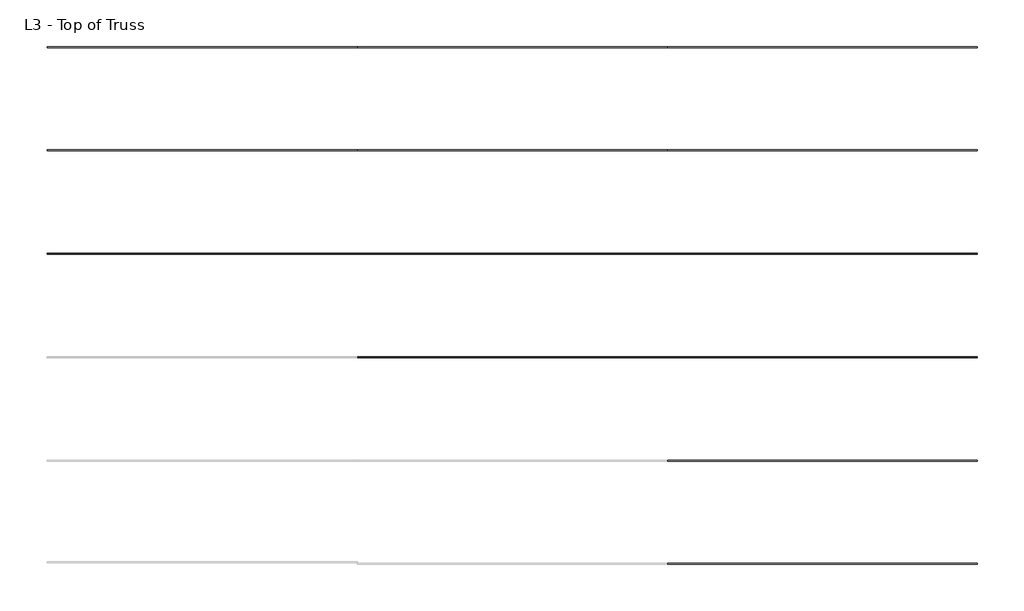
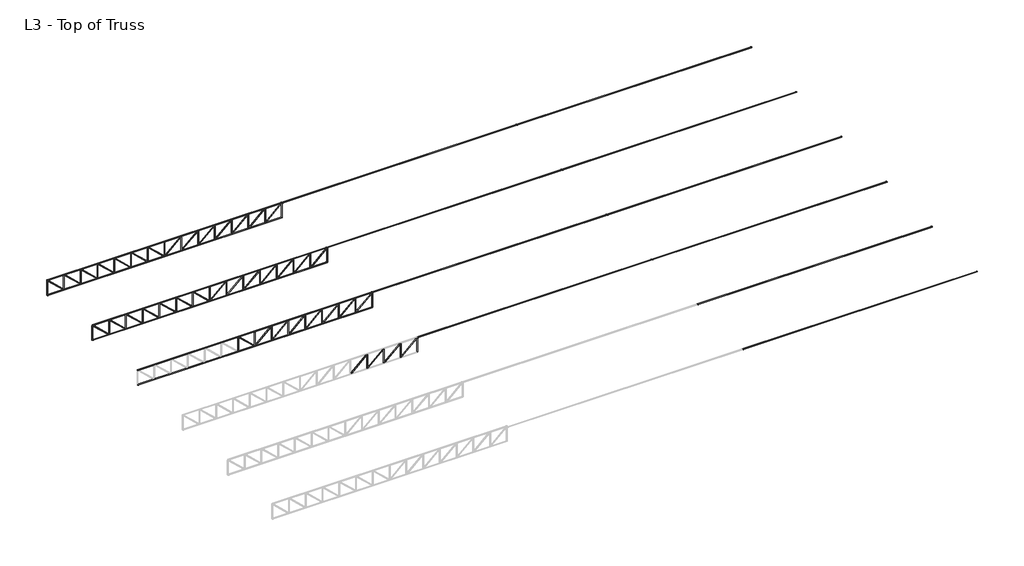
# One storey, part 2 of 2: 100 beams.
"""IFC4 building model written with IfcOpenShell, lengths in millimetres."""

import ifcopenshell
import ifcopenshell.guid

model = None  # the IFC model being written
_history = None  # IfcOwnerHistory: only IFC2X3 demands one
_inside = {}  # id of a spatial element -> (the spatial element, [elements in it])
_under = {}  # id of a project, library or spatial element -> (it, [spatial elements below it])
_declared = {}  # id of a project -> (the project, [libraries it declares])
_typed = {}  # id of a type object -> (the type object, [elements of that type])
_made_of = {}  # id of a material, layer set ... -> (it, [elements and type objects made of it])


def new_model(schema):
    """Start an empty IFC model of exactly this schema.

    Asked for "IFC4X3", IfcOpenShell would pick the latest addendum, in which some entities
    have other attributes; the version numbers below select the first issue.
    IFC2X3 requires an IfcOwnerHistory on every rooted entity: one is made here for all.
    """
    global model, _history
    if schema == "IFC4X3":
        model = ifcopenshell.file(schema_version=(4, 3, 0, 0))
    else:
        model = ifcopenshell.file(schema=schema)
    _inside.clear()
    _under.clear()
    _declared.clear()
    _typed.clear()
    _made_of.clear()
    _history = None
    if model.schema == "IFC2X3":
        org = make("IfcOrganization", Name="unknown")
        user = make(
            "IfcPersonAndOrganization",
            ThePerson=make("IfcPerson", FamilyName="unknown"),
            TheOrganization=org,
        )
        app = make(
            "IfcApplication",
            ApplicationDeveloper=org,
            Version="unknown",
            ApplicationFullName="unknown",
            ApplicationIdentifier="unknown",
        )
        _history = make(
            "IfcOwnerHistory",
            OwningUser=user,
            OwningApplication=app,
            ChangeAction="ADDED",
            CreationDate=0,
        )
    return model


def make(cls, **values):
    """One entity of the class cls with the attributes given. An attribute that is None is left unset."""
    return model.create_entity(
        cls, **{name: value for name, value in values.items() if value is not None}
    )


def rooted(cls, **values):
    """An entity with a GlobalId (a new one), such as an element, a storey or a relation."""
    return make(cls, GlobalId=ifcopenshell.guid.new(), OwnerHistory=_history, **values)


def si_unit(unit_type, name, prefix=None):
    """IfcSIUnit, for example si_unit("LENGTHUNIT", "METRE", prefix="MILLI")."""
    return make("IfcSIUnit", UnitType=unit_type, Prefix=prefix, Name=name)


def assignment(units):
    """IfcUnitAssignment: the units of a project."""
    return None if units is None else make("IfcUnitAssignment", Units=units)


def point(xyz):
    """IfcCartesianPoint."""
    return None if xyz is None else make("IfcCartesianPoint", Coordinates=xyz)


def direction(xyz):
    """IfcDirection."""
    return None if xyz is None else make("IfcDirection", DirectionRatios=xyz)


def frame(location, z_axis=None, x_axis=None):
    """IfcAxis2Placement3D, a coordinate frame: its origin and axes. An axis left out is left unset."""
    return make(
        "IfcAxis2Placement3D",
        Location=point(location),
        Axis=direction(z_axis),
        RefDirection=direction(x_axis),
    )


def frame_2d(location, x_axis=None):
    """IfcAxis2Placement2D, a coordinate frame in the plane: its origin and x axis."""
    return make(
        "IfcAxis2Placement2D", Location=point(location), RefDirection=direction(x_axis)
    )


def origin():
    """The frame at (0, 0, 0) with its axes left unset."""
    return frame((0.0, 0.0, 0.0))


def origin_2d():
    """The frame at (0, 0) in the plane with its x axis left unset."""
    return frame_2d((0.0, 0.0))


def place(relative_to, where):
    """IfcLocalPlacement: puts the frame where relative to a parent placement (None: the world)."""
    return make(
        "IfcLocalPlacement", PlacementRelTo=relative_to, RelativePlacement=where
    )


def context(
    kind, dimensions, precision=None, world=None, true_north=None, identifier=None
):
    """IfcGeometricRepresentationContext, for example the 3D "Model" context."""
    return make(
        "IfcGeometricRepresentationContext",
        ContextIdentifier=identifier,
        ContextType=kind,
        CoordinateSpaceDimension=dimensions,
        Precision=precision,
        WorldCoordinateSystem=world,
        TrueNorth=true_north,
    )


def project(units=None, contexts=None):
    """IfcProject with its units and contexts."""
    return rooted(
        "IfcProject",
        Name="project",
        RepresentationContexts=contexts,
        UnitsInContext=assignment(units),
    )


def spatial(cls, under=None, at=None, **own):
    """A site, building, storey or space (cls), placed at a placement, below another one or the project."""
    s = rooted(cls, ObjectPlacement=at, **own)
    if under is not None:
        _under.setdefault(under.id(), (under, []))[1].append(s)
    return s


def circle_curve(where, radius):
    """IfcCircle in the frame where."""
    return make("IfcCircle", Position=where, Radius=radius)


def trimmed(basis, trim1, trim2, sense, master):
    """IfcTrimmedCurve: the piece of a basis curve between two trims."""
    return make(
        "IfcTrimmedCurve",
        BasisCurve=basis,
        Trim1=trim1,
        Trim2=trim2,
        SenseAgreement=sense,
        MasterRepresentation=master,
    )


def segment(curve, same_sense, transition):
    """IfcCompositeCurveSegment."""
    return make(
        "IfcCompositeCurveSegment",
        Transition=transition,
        SameSense=same_sense,
        ParentCurve=curve,
    )


def composite_curve(segments, self_intersect=None):
    """IfcCompositeCurve: segments joined end to end."""
    return make("IfcCompositeCurve", Segments=segments, SelfIntersect=self_intersect)


def outline(outer, holes=None, kind="AREA"):
    """IfcArbitraryClosedProfileDef: a profile drawn as a closed curve; with holes, ...WithVoids."""
    if holes is None:
        return make("IfcArbitraryClosedProfileDef", ProfileType=kind, OuterCurve=outer)
    return make(
        "IfcArbitraryProfileDefWithVoids",
        ProfileType=kind,
        OuterCurve=outer,
        InnerCurves=holes,
    )


def extrude(swept, where, along, depth):
    """IfcExtrudedAreaSolid: the profile swept, set in the frame where, extruded along a direction by depth."""
    return make(
        "IfcExtrudedAreaSolid",
        SweptArea=swept,
        Position=where,
        ExtrudedDirection=direction(along),
        Depth=depth,
    )


def shape(context_of_items, identifier, shape_type, items):
    """IfcShapeRepresentation: the items that make up one representation, for example the "Body"."""
    return make(
        "IfcShapeRepresentation",
        ContextOfItems=context_of_items,
        RepresentationIdentifier=identifier,
        RepresentationType=shape_type,
        Items=items,
    )


def source(mapping_origin, context_of_items, identifier, shape_type, items):
    """IfcRepresentationMap: a shape defined once, which mapped items show again and again."""
    return make(
        "IfcRepresentationMap",
        MappingOrigin=mapping_origin,
        MappedRepresentation=shape(context_of_items, identifier, shape_type, items),
    )


def transform(
    local_origin,
    x_axis=None,
    y_axis=None,
    z_axis=None,
    scale=None,
    scale2=None,
    scale3=None,
    uniform=True,
):
    """IfcCartesianTransformationOperator3D, or its non-uniform kind. x_axis, y_axis, z_axis: its Axis1, 2, 3."""
    if uniform:
        return make(
            "IfcCartesianTransformationOperator3D",
            Axis1=direction(x_axis),
            Axis2=direction(y_axis),
            LocalOrigin=point(local_origin),
            Scale=scale,
            Axis3=direction(z_axis),
        )
    return make(
        "IfcCartesianTransformationOperator3DnonUniform",
        Axis1=direction(x_axis),
        Axis2=direction(y_axis),
        LocalOrigin=point(local_origin),
        Scale=scale,
        Axis3=direction(z_axis),
        Scale2=scale2,
        Scale3=scale3,
    )


def mapped(mapping_source, mapping_target):
    """IfcMappedItem: shows the shape of a source again, moved by a transform."""
    return make(
        "IfcMappedItem", MappingSource=mapping_source, MappingTarget=mapping_target
    )


def made_of(thing, what):
    """Note that an element or type object is made of a material, layer set ...; save() writes the relation."""
    if what is not None:
        _made_of.setdefault(what.id(), (what, []))[1].append(thing)
    return thing


def element(
    cls,
    number,
    at=None,
    inside=None,
    cuts=None,
    type_object=None,
    material=None,
    context=None,
    identifier="Body",
    shape_type=None,
    held_by="IfcProductDefinitionShape",
    body=None,
    shapes=None,
    **own,
):
    """One element of the class cls, such as IfcWall. Its Tag is "e" and its number.

    at: its placement. inside: the storey or other place that contains it. cuts: it is an
    opening in that element (IfcRelVoidsElement). A single representation is given by context,
    identifier, shape_type and body (its items); several are given by shapes. held_by: the class
    of the entity that holds the representations. save() writes the other relations.
    """
    e = rooted(cls, Tag="e%d" % number, ObjectPlacement=at, **own)
    if body is not None:
        shapes = [shape(context, identifier, shape_type, body)]
    if shapes is not None:
        e.Representation = make(held_by, Representations=shapes)
    if inside is not None:
        _inside.setdefault(inside.id(), (inside, []))[1].append(e)
    if cuts is not None:
        rooted(
            "IfcRelVoidsElement", RelatingBuildingElement=cuts, RelatedOpeningElement=e
        )
    if type_object is not None:
        _typed.setdefault(type_object.id(), (type_object, []))[1].append(e)
    return made_of(e, material)


def aggregate(whole, parts):
    """IfcRelAggregates: a whole, such as a stair, and the parts it consists of."""
    return rooted("IfcRelAggregates", RelatingObject=whole, RelatedObjects=parts)


def save(model, path):
    """Write the relations noted so far, then the file.

    IfcRelAggregates (storeys below a building ...), IfcRelContainedInSpatialStructure (elements
    in a storey), IfcRelDefinesByType, IfcRelAssociatesMaterial and IfcRelDeclares: one each for
    every whole, place, type object, material and project.
    """
    for whole, parts in _under.values():
        aggregate(whole, parts)
    for where, things in _inside.values():
        rooted(
            "IfcRelContainedInSpatialStructure",
            RelatedElements=things,
            RelatingStructure=where,
        )
    for kind, things in _typed.values():
        rooted("IfcRelDefinesByType", RelatedObjects=things, RelatingType=kind)
    for what, things in _made_of.values():
        rooted("IfcRelAssociatesMaterial", RelatedObjects=things, RelatingMaterial=what)
    for by, libraries in _declared.values():
        rooted("IfcRelDeclares", RelatingContext=by, RelatedDefinitions=libraries)
    model.write(path)


def circular_hollow_sections_chs60_3x5_c94bd862(model_context):
    return source(origin(), model_context, "Body", "SweptSolid", [
        extrude(outline(composite_curve([segment(trimmed(circle_curve(origin_2d(), 30.15), [point((-30.15, 0.0))], [point((30.15, 0.0))], False, "CARTESIAN"), True, "CONTINUOUS"), segment(trimmed(circle_curve(origin_2d(), 30.15), [point((30.15, 0.0))], [point((-30.15, 0.0))], False, "CARTESIAN"), True, "CONTINUOUS")], self_intersect=False), holes=[composite_curve([segment(trimmed(circle_curve(origin_2d(), 25.15), [point((25.15, 0.0))], [point((-25.15, 0.0))], True, "CARTESIAN"), True, "CONTINUOUS"), segment(trimmed(circle_curve(origin_2d(), 25.15), [point((-25.15, 0.0))], [point((25.15, 0.0))], True, "CARTESIAN"), True, "CONTINUOUS")], self_intersect=False)]), frame((-557.0, 0.0, 0.0), z_axis=(1.0, 0.0, 0.0), x_axis=(0.0, 1.0, 0.0)), (0.0, 0.0, 1.0), 1114.0),
    ])


def circular_hollow_sections_chs60_3x5_b8a643cb(model_context):
    return source(origin(), model_context, "Body", "SweptSolid", [
        extrude(outline(composite_curve([segment(trimmed(circle_curve(origin_2d(), 30.15), [point((-30.15, 0.0))], [point((30.15, 0.0))], False, "CARTESIAN"), True, "CONTINUOUS"), segment(trimmed(circle_curve(origin_2d(), 30.15), [point((30.15, 0.0))], [point((-30.15, 0.0))], False, "CARTESIAN"), True, "CONTINUOUS")], self_intersect=False), holes=[composite_curve([segment(trimmed(circle_curve(origin_2d(), 25.15), [point((25.15, 0.0))], [point((-25.15, 0.0))], True, "CARTESIAN"), True, "CONTINUOUS"), segment(trimmed(circle_curve(origin_2d(), 25.15), [point((-25.15, 0.0))], [point((25.15, 0.0))], True, "CARTESIAN"), True, "CONTINUOUS")], self_intersect=False)]), frame((-790.0, 0.0, 0.0), z_axis=(1.0, 0.0, 0.0), x_axis=(0.0, 1.0, 0.0)), (0.0, 0.0, 1.0), 1580.0),
    ])


def circular_hollow_sections_chs60_3x5_ee2473de(model_context):
    return source(origin(), model_context, "Body", "SweptSolid", [
        extrude(outline(composite_curve([segment(trimmed(circle_curve(origin_2d(), 30.15), [point((-30.15, 0.0))], [point((30.15, 0.0))], False, "CARTESIAN"), True, "CONTINUOUS"), segment(trimmed(circle_curve(origin_2d(), 30.15), [point((30.15, 0.0))], [point((-30.15, 0.0))], False, "CARTESIAN"), True, "CONTINUOUS")], self_intersect=False), holes=[composite_curve([segment(trimmed(circle_curve(origin_2d(), 25.15), [point((25.15, 0.0))], [point((-25.15, 0.0))], True, "CARTESIAN"), True, "CONTINUOUS"), segment(trimmed(circle_curve(origin_2d(), 25.15), [point((-25.15, 0.0))], [point((25.15, 0.0))], True, "CARTESIAN"), True, "CONTINUOUS")], self_intersect=False)]), frame((-9000.0, 0.0, 0.0), z_axis=(1.0, 0.0, 0.0), x_axis=(0.0, 1.0, 0.0)), (0.0, 0.0, 1.0), 18000.0),
    ])


def circular_hollow_sections_chs60_3x5_7809bf4e(model_context):
    return source(origin(), model_context, "Body", "SweptSolid", [
        extrude(outline(composite_curve([segment(trimmed(circle_curve(origin_2d(), 30.15), [point((-30.15, 0.0))], [point((30.15, 0.0))], False, "CARTESIAN"), True, "CONTINUOUS"), segment(trimmed(circle_curve(origin_2d(), 30.15), [point((30.15, 0.0))], [point((-30.15, 0.0))], False, "CARTESIAN"), True, "CONTINUOUS")], self_intersect=False), holes=[composite_curve([segment(trimmed(circle_curve(origin_2d(), 25.15), [point((25.15, 0.0))], [point((-25.15, 0.0))], True, "CARTESIAN"), True, "CONTINUOUS"), segment(trimmed(circle_curve(origin_2d(), 25.15), [point((-25.15, 0.0))], [point((25.15, 0.0))], True, "CARTESIAN"), True, "CONTINUOUS")], self_intersect=False)]), frame((-600.0, 0.0, 0.0), z_axis=(1.0, 0.0, 0.0), x_axis=(0.0, 1.0, 0.0)), (0.0, 0.0, 1.0), 1157.0),
    ])


model = new_model("IFC4")

# Units and contexts
model_context = context("Model", 3, world=origin())
ifc_project = project(units=[si_unit("LENGTHUNIT", "METRE", prefix="MILLI")], contexts=[model_context])

# Site, building, storey
site = spatial("IfcSite", under=ifc_project)
building = spatial("IfcBuilding", under=site)
storey = spatial("IfcBuildingStorey", under=building, Name="L3 - Top of Truss", Elevation=7800.0)

# Beams
placement = place(None, origin())
circular_hollow_sections_chs60_3x5_shape = circular_hollow_sections_chs60_3x5_c94bd862(model_context)
element("IfcBeam", 1, ObjectType="Circular Hollow Sections : CHS60.3x5", at=placement, inside=storey, context=model_context, shape_type="MappedRepresentation", body=[
    mapped(circular_hollow_sections_chs60_3x5_shape, transform((9574.7303686, 941.2380918, 7200.0), x_axis=(0.0, 0.0, 1.0), y_axis=(0.0, -1.0, 0.0), z_axis=(1.0, 0.0, 0.0))),
])
element("IfcBeam", 2, ObjectType="Circular Hollow Sections : CHS60.3x5", at=placement, inside=storey, context=model_context, shape_type="MappedRepresentation", body=[
    mapped(circular_hollow_sections_chs60_3x5_shape, transform((-5853.84106, 941.2380918, 7200.0), x_axis=(0.0, 0.0, 1.0), y_axis=(0.0, -1.0, 0.0), z_axis=(1.0, 0.0, 0.0))),
])
element("IfcBeam", 3, ObjectType="Circular Hollow Sections : CHS60.3x5", at=placement, inside=storey, context=model_context, shape_type="MappedRepresentation", body=[
    mapped(circular_hollow_sections_chs60_3x5_shape, transform((8289.0160829, 941.2380918, 7200.0), x_axis=(0.0, 0.0, 1.0), y_axis=(0.0, -1.0, 0.0), z_axis=(1.0, 0.0, 0.0))),
])
element("IfcBeam", 4, ObjectType="Circular Hollow Sections : CHS60.3x5", at=placement, inside=storey, context=model_context, shape_type="MappedRepresentation", body=[
    mapped(circular_hollow_sections_chs60_3x5_shape, transform((-4568.1267743, 941.2380918, 7200.0), x_axis=(0.0, 0.0, 1.0), y_axis=(0.0, -1.0, 0.0), z_axis=(1.0, 0.0, 0.0))),
])
element("IfcBeam", 5, ObjectType="Circular Hollow Sections : CHS60.3x5", at=placement, inside=storey, context=model_context, shape_type="MappedRepresentation", body=[
    mapped(circular_hollow_sections_chs60_3x5_shape, transform((7003.3017972, 941.2380918, 7200.0), x_axis=(0.0, 0.0, 1.0), y_axis=(0.0, -1.0, 0.0), z_axis=(1.0, 0.0, 0.0))),
])
element("IfcBeam", 6, ObjectType="Circular Hollow Sections : CHS60.3x5", at=placement, inside=storey, context=model_context, shape_type="MappedRepresentation", body=[
    mapped(circular_hollow_sections_chs60_3x5_shape, transform((-3282.4124885, 941.2380918, 7200.0), x_axis=(0.0, 0.0, 1.0), y_axis=(0.0, -1.0, 0.0), z_axis=(1.0, 0.0, 0.0))),
])
element("IfcBeam", 7, ObjectType="Circular Hollow Sections : CHS60.3x5", at=placement, inside=storey, context=model_context, shape_type="MappedRepresentation", body=[
    mapped(circular_hollow_sections_chs60_3x5_shape, transform((5717.5875115, 941.2380918, 7200.0), x_axis=(0.0, 0.0, 1.0), y_axis=(0.0, -1.0, 0.0), z_axis=(1.0, 0.0, 0.0))),
])
element("IfcBeam", 8, ObjectType="Circular Hollow Sections : CHS60.3x5", at=placement, inside=storey, context=model_context, shape_type="MappedRepresentation", body=[
    mapped(circular_hollow_sections_chs60_3x5_shape, transform((4431.8732257, 941.2380918, 7200.0), x_axis=(0.0, 0.0, 1.0), y_axis=(0.0, -1.0, 0.0), z_axis=(1.0, 0.0, 0.0))),
])
element("IfcBeam", 9, ObjectType="Circular Hollow Sections : CHS60.3x5", at=placement, inside=storey, context=model_context, shape_type="MappedRepresentation", body=[
    mapped(circular_hollow_sections_chs60_3x5_shape, transform((3146.15894, 941.2380918, 7200.0), x_axis=(0.0, 0.0, 1.0), y_axis=(0.0, -1.0, 0.0), z_axis=(1.0, 0.0, 0.0))),
])
element("IfcBeam", 10, ObjectType="Circular Hollow Sections : CHS60.3x5", at=placement, inside=storey, context=model_context, shape_type="MappedRepresentation", body=[
    mapped(circular_hollow_sections_chs60_3x5_shape, transform((-1996.6982028, 941.2380918, 7200.0), x_axis=(0.0, 0.0, 1.0), y_axis=(0.0, -1.0, 0.0), z_axis=(1.0, 0.0, 0.0))),
])
element("IfcBeam", 11, ObjectType="Circular Hollow Sections : CHS60.3x5", at=placement, inside=storey, context=model_context, shape_type="MappedRepresentation", body=[
    mapped(circular_hollow_sections_chs60_3x5_shape, transform((-710.9839171, 941.2380918, 7200.0), x_axis=(0.0, 0.0, 1.0), y_axis=(0.0, -1.0, 0.0), z_axis=(1.0, 0.0, 0.0))),
])
element("IfcBeam", 12, ObjectType="Circular Hollow Sections : CHS60.3x5", at=placement, inside=storey, context=model_context, shape_type="MappedRepresentation", body=[
    mapped(circular_hollow_sections_chs60_3x5_shape, transform((574.7303686, 941.2380918, 7200.0), x_axis=(0.0, 0.0, 1.0), y_axis=(0.0, -1.0, 0.0), z_axis=(1.0, 0.0, 0.0))),
])
element("IfcBeam", 13, ObjectType="Circular Hollow Sections : CHS60.3x5", at=placement, inside=storey, context=model_context, shape_type="MappedRepresentation", body=[
    mapped(circular_hollow_sections_chs60_3x5_shape, transform((1860.4446543, 941.2380918, 7200.0), x_axis=(0.0, 0.0, 1.0), y_axis=(0.0, -1.0, 0.0), z_axis=(1.0, 0.0, 0.0))),
])
element("IfcBeam", 14, ObjectType="Circular Hollow Sections : CHS60.3x5", at=placement, inside=storey, context=model_context, shape_type="MappedRepresentation", body=[
    mapped(circular_hollow_sections_chs60_3x5_shape, transform((9574.7303686, 6941.2380918, 7200.0), x_axis=(0.0, 0.0, 1.0), y_axis=(0.0, -1.0, 0.0), z_axis=(1.0, 0.0, 0.0))),
])
element("IfcBeam", 15, ObjectType="Circular Hollow Sections : CHS60.3x5", at=placement, inside=storey, context=model_context, shape_type="MappedRepresentation", body=[
    mapped(circular_hollow_sections_chs60_3x5_shape, transform((-5853.84106, 6941.2380918, 7200.0), x_axis=(0.0, 0.0, 1.0), y_axis=(0.0, -1.0, 0.0), z_axis=(1.0, 0.0, 0.0))),
])
element("IfcBeam", 16, ObjectType="Circular Hollow Sections : CHS60.3x5", at=placement, inside=storey, context=model_context, shape_type="MappedRepresentation", body=[
    mapped(circular_hollow_sections_chs60_3x5_shape, transform((8289.0160829, 6941.2380918, 7200.0), x_axis=(0.0, 0.0, 1.0), y_axis=(0.0, -1.0, 0.0), z_axis=(1.0, 0.0, 0.0))),
])
element("IfcBeam", 17, ObjectType="Circular Hollow Sections : CHS60.3x5", at=placement, inside=storey, context=model_context, shape_type="MappedRepresentation", body=[
    mapped(circular_hollow_sections_chs60_3x5_shape, transform((-4568.1267743, 6941.2380918, 7200.0), x_axis=(0.0, 0.0, 1.0), y_axis=(0.0, -1.0, 0.0), z_axis=(1.0, 0.0, 0.0))),
])
element("IfcBeam", 18, ObjectType="Circular Hollow Sections : CHS60.3x5", at=placement, inside=storey, context=model_context, shape_type="MappedRepresentation", body=[
    mapped(circular_hollow_sections_chs60_3x5_shape, transform((7003.3017972, 6941.2380918, 7200.0), x_axis=(0.0, 0.0, 1.0), y_axis=(0.0, -1.0, 0.0), z_axis=(1.0, 0.0, 0.0))),
])
element("IfcBeam", 19, ObjectType="Circular Hollow Sections : CHS60.3x5", at=placement, inside=storey, context=model_context, shape_type="MappedRepresentation", body=[
    mapped(circular_hollow_sections_chs60_3x5_shape, transform((-3282.4124885, 6941.2380918, 7200.0), x_axis=(0.0, 0.0, 1.0), y_axis=(0.0, -1.0, 0.0), z_axis=(1.0, 0.0, 0.0))),
])
element("IfcBeam", 20, ObjectType="Circular Hollow Sections : CHS60.3x5", at=placement, inside=storey, context=model_context, shape_type="MappedRepresentation", body=[
    mapped(circular_hollow_sections_chs60_3x5_shape, transform((5717.5875115, 6941.2380918, 7200.0), x_axis=(0.0, 0.0, 1.0), y_axis=(0.0, -1.0, 0.0), z_axis=(1.0, 0.0, 0.0))),
])
element("IfcBeam", 21, ObjectType="Circular Hollow Sections : CHS60.3x5", at=placement, inside=storey, context=model_context, shape_type="MappedRepresentation", body=[
    mapped(circular_hollow_sections_chs60_3x5_shape, transform((4431.8732257, 6941.2380918, 7200.0), x_axis=(0.0, 0.0, 1.0), y_axis=(0.0, -1.0, 0.0), z_axis=(1.0, 0.0, 0.0))),
])
element("IfcBeam", 22, ObjectType="Circular Hollow Sections : CHS60.3x5", at=placement, inside=storey, context=model_context, shape_type="MappedRepresentation", body=[
    mapped(circular_hollow_sections_chs60_3x5_shape, transform((3146.15894, 6941.2380918, 7200.0), x_axis=(0.0, 0.0, 1.0), y_axis=(0.0, -1.0, 0.0), z_axis=(1.0, 0.0, 0.0))),
])
element("IfcBeam", 23, ObjectType="Circular Hollow Sections : CHS60.3x5", at=placement, inside=storey, context=model_context, shape_type="MappedRepresentation", body=[
    mapped(circular_hollow_sections_chs60_3x5_shape, transform((-1996.6982028, 6941.2380918, 7200.0), x_axis=(0.0, 0.0, 1.0), y_axis=(0.0, -1.0, 0.0), z_axis=(1.0, 0.0, 0.0))),
])
element("IfcBeam", 24, ObjectType="Circular Hollow Sections : CHS60.3x5", at=placement, inside=storey, context=model_context, shape_type="MappedRepresentation", body=[
    mapped(circular_hollow_sections_chs60_3x5_shape, transform((-710.9839171, 6941.2380918, 7200.0), x_axis=(0.0, 0.0, 1.0), y_axis=(0.0, -1.0, 0.0), z_axis=(1.0, 0.0, 0.0))),
])
element("IfcBeam", 25, ObjectType="Circular Hollow Sections : CHS60.3x5", at=placement, inside=storey, context=model_context, shape_type="MappedRepresentation", body=[
    mapped(circular_hollow_sections_chs60_3x5_shape, transform((574.7303686, 6941.2380918, 7200.0), x_axis=(0.0, 0.0, 1.0), y_axis=(0.0, -1.0, 0.0), z_axis=(1.0, 0.0, 0.0))),
])
element("IfcBeam", 26, ObjectType="Circular Hollow Sections : CHS60.3x5", at=placement, inside=storey, context=model_context, shape_type="MappedRepresentation", body=[
    mapped(circular_hollow_sections_chs60_3x5_shape, transform((1860.4446543, 6941.2380918, 7200.0), x_axis=(0.0, 0.0, 1.0), y_axis=(0.0, -1.0, 0.0), z_axis=(1.0, 0.0, 0.0))),
])
element("IfcBeam", 27, ObjectType="Circular Hollow Sections : CHS60.3x5", at=placement, inside=storey, context=model_context, shape_type="MappedRepresentation", body=[
    mapped(circular_hollow_sections_chs60_3x5_shape, transform((9574.7303686, -5058.7619082, 7200.0), x_axis=(0.0, 0.0, 1.0), y_axis=(0.0, -1.0, 0.0), z_axis=(1.0, 0.0, 0.0))),
])
element("IfcBeam", 28, ObjectType="Circular Hollow Sections : CHS60.3x5", at=placement, inside=storey, context=model_context, shape_type="MappedRepresentation", body=[
    mapped(circular_hollow_sections_chs60_3x5_shape, transform((8289.0160829, -5058.7619082, 7200.0), x_axis=(0.0, 0.0, 1.0), y_axis=(0.0, -1.0, 0.0), z_axis=(1.0, 0.0, 0.0))),
])
element("IfcBeam", 29, ObjectType="Circular Hollow Sections : CHS60.3x5", at=placement, inside=storey, context=model_context, shape_type="MappedRepresentation", body=[
    mapped(circular_hollow_sections_chs60_3x5_shape, transform((7003.3017972, -5058.7619082, 7200.0), x_axis=(0.0, 0.0, 1.0), y_axis=(0.0, -1.0, 0.0), z_axis=(1.0, 0.0, 0.0))),
])
element("IfcBeam", 30, ObjectType="Circular Hollow Sections : CHS60.3x5", at=placement, inside=storey, context=model_context, shape_type="MappedRepresentation", body=[
    mapped(circular_hollow_sections_chs60_3x5_shape, transform((5717.5875115, -5058.7619082, 7200.0), x_axis=(0.0, 0.0, 1.0), y_axis=(0.0, -1.0, 0.0), z_axis=(1.0, 0.0, 0.0))),
])
element("IfcBeam", 31, ObjectType="Circular Hollow Sections : CHS60.3x5", at=placement, inside=storey, context=model_context, shape_type="MappedRepresentation", body=[
    mapped(circular_hollow_sections_chs60_3x5_shape, transform((4431.8732257, -5058.7619082, 7200.0), x_axis=(0.0, 0.0, 1.0), y_axis=(0.0, -1.0, 0.0), z_axis=(1.0, 0.0, 0.0))),
])
element("IfcBeam", 32, ObjectType="Circular Hollow Sections : CHS60.3x5", at=placement, inside=storey, context=model_context, shape_type="MappedRepresentation", body=[
    mapped(circular_hollow_sections_chs60_3x5_shape, transform((3146.15894, -5058.7619082, 7200.0), x_axis=(0.0, 0.0, 1.0), y_axis=(0.0, -1.0, 0.0), z_axis=(1.0, 0.0, 0.0))),
])
element("IfcBeam", 33, ObjectType="Circular Hollow Sections : CHS60.3x5", at=placement, inside=storey, context=model_context, shape_type="MappedRepresentation", body=[
    mapped(circular_hollow_sections_chs60_3x5_shape, transform((574.7303686, -5058.7619082, 7200.0), x_axis=(0.0, 0.0, 1.0), y_axis=(0.0, -1.0, 0.0), z_axis=(1.0, 0.0, 0.0))),
])
element("IfcBeam", 34, ObjectType="Circular Hollow Sections : CHS60.3x5", at=placement, inside=storey, context=model_context, shape_type="MappedRepresentation", body=[
    mapped(circular_hollow_sections_chs60_3x5_shape, transform((1860.4446543, -5058.7619082, 7200.0), x_axis=(0.0, 0.0, 1.0), y_axis=(0.0, -1.0, 0.0), z_axis=(1.0, 0.0, 0.0))),
])
element("IfcBeam", 35, ObjectType="Circular Hollow Sections : CHS60.3x5", at=placement, inside=storey, context=model_context, shape_type="MappedRepresentation", body=[
    mapped(circular_hollow_sections_chs60_3x5_shape, transform((9574.7303686, -11058.7619082, 7200.0), x_axis=(0.0, 0.0, 1.0), y_axis=(0.0, -1.0, 0.0), z_axis=(1.0, 0.0, 0.0))),
])
element("IfcBeam", 36, ObjectType="Circular Hollow Sections : CHS60.3x5", at=placement, inside=storey, context=model_context, shape_type="MappedRepresentation", body=[
    mapped(circular_hollow_sections_chs60_3x5_shape, transform((8289.0160829, -11058.7619082, 7200.0), x_axis=(0.0, 0.0, 1.0), y_axis=(0.0, -1.0, 0.0), z_axis=(1.0, 0.0, 0.0))),
])
element("IfcBeam", 37, ObjectType="Circular Hollow Sections : CHS60.3x5", at=placement, inside=storey, context=model_context, shape_type="MappedRepresentation", body=[
    mapped(circular_hollow_sections_chs60_3x5_shape, transform((7003.3017972, -11058.7619082, 7200.0), x_axis=(0.0, 0.0, 1.0), y_axis=(0.0, -1.0, 0.0), z_axis=(1.0, 0.0, 0.0))),
])
circular_hollow_sections_chs60_3x5_2_shape = circular_hollow_sections_chs60_3x5_b8a643cb(model_context)
element("IfcBeam", 38, ObjectType="Circular Hollow Sections : CHS60.3x5", at=placement, inside=storey, context=model_context, shape_type="MappedRepresentation", body=[
    mapped(circular_hollow_sections_chs60_3x5_2_shape, transform((8931.8732257, 941.2380918, 7200.0), x_axis=(0.7310552682428691, 0.0, 0.6823182503600111), y_axis=(0.0, -1.0, 0.0), z_axis=(0.6823182503600111, 0.0, -0.7310552682428691))),
])
element("IfcBeam", 39, ObjectType="Circular Hollow Sections : CHS60.3x5", at=placement, inside=storey, context=model_context, shape_type="MappedRepresentation", body=[
    mapped(circular_hollow_sections_chs60_3x5_2_shape, transform((-5210.9839171, 941.2380918, 7200.0), x_axis=(0.7310552682428689, 0.0, -0.6823182503600113), y_axis=(0.0, -1.0, 0.0), z_axis=(-0.6823182503600113, 0.0, -0.7310552682428689))),
])
element("IfcBeam", 40, ObjectType="Circular Hollow Sections : CHS60.3x5", at=placement, inside=storey, context=model_context, shape_type="MappedRepresentation", body=[
    mapped(circular_hollow_sections_chs60_3x5_2_shape, transform((7646.15894, 941.2380918, 7200.0), x_axis=(0.7310552682428691, 0.0, 0.6823182503600111), y_axis=(0.0, -1.0, 0.0), z_axis=(0.6823182503600111, 0.0, -0.7310552682428691))),
])
element("IfcBeam", 41, ObjectType="Circular Hollow Sections : CHS60.3x5", at=placement, inside=storey, context=model_context, shape_type="MappedRepresentation", body=[
    mapped(circular_hollow_sections_chs60_3x5_2_shape, transform((-3925.2696314, 941.2380918, 7200.0), x_axis=(0.7310552682428689, 0.0, -0.6823182503600113), y_axis=(0.0, -1.0, 0.0), z_axis=(-0.6823182503600113, 0.0, -0.7310552682428689))),
])
element("IfcBeam", 42, ObjectType="Circular Hollow Sections : CHS60.3x5", at=placement, inside=storey, context=model_context, shape_type="MappedRepresentation", body=[
    mapped(circular_hollow_sections_chs60_3x5_2_shape, transform((6360.4446543, 941.2380918, 7200.0), x_axis=(0.7310552682428691, 0.0, 0.6823182503600111), y_axis=(0.0, -1.0, 0.0), z_axis=(0.6823182503600111, 0.0, -0.7310552682428691))),
])
element("IfcBeam", 43, ObjectType="Circular Hollow Sections : CHS60.3x5", at=placement, inside=storey, context=model_context, shape_type="MappedRepresentation", body=[
    mapped(circular_hollow_sections_chs60_3x5_2_shape, transform((-2639.5553457, 941.2380918, 7200.0), x_axis=(0.7310552682428689, 0.0, -0.6823182503600113), y_axis=(0.0, -1.0, 0.0), z_axis=(-0.6823182503600113, 0.0, -0.7310552682428689))),
])
element("IfcBeam", 44, ObjectType="Circular Hollow Sections : CHS60.3x5", at=placement, inside=storey, context=model_context, shape_type="MappedRepresentation", body=[
    mapped(circular_hollow_sections_chs60_3x5_2_shape, transform((5074.7303686, 941.2380918, 7200.0), x_axis=(0.7310552682428691, 0.0, 0.6823182503600111), y_axis=(0.0, -1.0, 0.0), z_axis=(0.6823182503600111, 0.0, -0.7310552682428691))),
])
element("IfcBeam", 45, ObjectType="Circular Hollow Sections : CHS60.3x5", at=placement, inside=storey, context=model_context, shape_type="MappedRepresentation", body=[
    mapped(circular_hollow_sections_chs60_3x5_2_shape, transform((3789.0160829, 941.2380918, 7200.0), x_axis=(0.7310552682428691, 0.0, 0.6823182503600111), y_axis=(0.0, -1.0, 0.0), z_axis=(0.6823182503600111, 0.0, -0.7310552682428691))),
])
element("IfcBeam", 46, ObjectType="Circular Hollow Sections : CHS60.3x5", at=placement, inside=storey, context=model_context, shape_type="MappedRepresentation", body=[
    mapped(circular_hollow_sections_chs60_3x5_2_shape, transform((10217.5875115, 941.2380918, 7200.0), x_axis=(0.7310552682428691, 0.0, 0.6823182503600111), y_axis=(0.0, -1.0, 0.0), z_axis=(0.6823182503600111, 0.0, -0.7310552682428691))),
])
element("IfcBeam", 47, ObjectType="Circular Hollow Sections : CHS60.3x5", at=placement, inside=storey, context=model_context, shape_type="MappedRepresentation", body=[
    mapped(circular_hollow_sections_chs60_3x5_2_shape, transform((2503.3017972, 941.2380918, 7200.0), x_axis=(0.7310552682428691, 0.0, 0.682318250360011), y_axis=(0.0, -1.0, 0.0), z_axis=(0.682318250360011, 0.0, -0.7310552682428691))),
])
element("IfcBeam", 48, ObjectType="Circular Hollow Sections : CHS60.3x5", at=placement, inside=storey, context=model_context, shape_type="MappedRepresentation", body=[
    mapped(circular_hollow_sections_chs60_3x5_2_shape, transform((-1353.84106, 941.2380918, 7200.0), x_axis=(0.7310552682428689, 0.0, -0.6823182503600113), y_axis=(0.0, -1.0, 0.0), z_axis=(-0.6823182503600113, 0.0, -0.7310552682428689))),
])
element("IfcBeam", 49, ObjectType="Circular Hollow Sections : CHS60.3x5", at=placement, inside=storey, context=model_context, shape_type="MappedRepresentation", body=[
    mapped(circular_hollow_sections_chs60_3x5_2_shape, transform((-68.1267743, 941.2380918, 7200.0), x_axis=(0.7310552682428689, 0.0, -0.6823182503600113), y_axis=(0.0, -1.0, 0.0), z_axis=(-0.6823182503600113, 0.0, -0.7310552682428689))),
])
element("IfcBeam", 50, ObjectType="Circular Hollow Sections : CHS60.3x5", at=placement, inside=storey, context=model_context, shape_type="MappedRepresentation", body=[
    mapped(circular_hollow_sections_chs60_3x5_2_shape, transform((-6496.6982028, 941.2380918, 7200.0), x_axis=(0.7310552682428688, 0.0, -0.6823182503600115), y_axis=(0.0, -1.0, 0.0), z_axis=(-0.6823182503600115, 0.0, -0.7310552682428688))),
])
element("IfcBeam", 51, ObjectType="Circular Hollow Sections : CHS60.3x5", at=placement, inside=storey, context=model_context, shape_type="MappedRepresentation", body=[
    mapped(circular_hollow_sections_chs60_3x5_2_shape, transform((1217.5875115, 941.2380918, 7200.0), x_axis=(0.7310552682428689, 0.0, -0.6823182503600113), y_axis=(0.0, -1.0, 0.0), z_axis=(-0.6823182503600113, 0.0, -0.7310552682428689))),
])
element("IfcBeam", 52, ObjectType="Circular Hollow Sections : CHS60.3x5", at=placement, inside=storey, context=model_context, shape_type="MappedRepresentation", body=[
    mapped(circular_hollow_sections_chs60_3x5_2_shape, transform((8931.8732257, 6941.2380918, 7200.0), x_axis=(0.7310552682428691, 0.0, 0.6823182503600111), y_axis=(0.0, -1.0, 0.0), z_axis=(0.6823182503600111, 0.0, -0.7310552682428691))),
])
element("IfcBeam", 53, ObjectType="Circular Hollow Sections : CHS60.3x5", at=placement, inside=storey, context=model_context, shape_type="MappedRepresentation", body=[
    mapped(circular_hollow_sections_chs60_3x5_2_shape, transform((-5210.9839171, 6941.2380918, 7200.0), x_axis=(0.7310552682428689, 0.0, -0.6823182503600113), y_axis=(0.0, -1.0, 0.0), z_axis=(-0.6823182503600113, 0.0, -0.7310552682428689))),
])
element("IfcBeam", 54, ObjectType="Circular Hollow Sections : CHS60.3x5", at=placement, inside=storey, context=model_context, shape_type="MappedRepresentation", body=[
    mapped(circular_hollow_sections_chs60_3x5_2_shape, transform((7646.15894, 6941.2380918, 7200.0), x_axis=(0.7310552682428691, 0.0, 0.6823182503600111), y_axis=(0.0, -1.0, 0.0), z_axis=(0.6823182503600111, 0.0, -0.7310552682428691))),
])
element("IfcBeam", 55, ObjectType="Circular Hollow Sections : CHS60.3x5", at=placement, inside=storey, context=model_context, shape_type="MappedRepresentation", body=[
    mapped(circular_hollow_sections_chs60_3x5_2_shape, transform((-3925.2696314, 6941.2380918, 7200.0), x_axis=(0.7310552682428689, 0.0, -0.6823182503600113), y_axis=(0.0, -1.0, 0.0), z_axis=(-0.6823182503600113, 0.0, -0.7310552682428689))),
])
element("IfcBeam", 56, ObjectType="Circular Hollow Sections : CHS60.3x5", at=placement, inside=storey, context=model_context, shape_type="MappedRepresentation", body=[
    mapped(circular_hollow_sections_chs60_3x5_2_shape, transform((6360.4446543, 6941.2380918, 7200.0), x_axis=(0.7310552682428691, 0.0, 0.6823182503600111), y_axis=(0.0, -1.0, 0.0), z_axis=(0.6823182503600111, 0.0, -0.7310552682428691))),
])
element("IfcBeam", 57, ObjectType="Circular Hollow Sections : CHS60.3x5", at=placement, inside=storey, context=model_context, shape_type="MappedRepresentation", body=[
    mapped(circular_hollow_sections_chs60_3x5_2_shape, transform((-2639.5553457, 6941.2380918, 7200.0), x_axis=(0.7310552682428689, 0.0, -0.6823182503600113), y_axis=(0.0, -1.0, 0.0), z_axis=(-0.6823182503600113, 0.0, -0.7310552682428689))),
])
element("IfcBeam", 58, ObjectType="Circular Hollow Sections : CHS60.3x5", at=placement, inside=storey, context=model_context, shape_type="MappedRepresentation", body=[
    mapped(circular_hollow_sections_chs60_3x5_2_shape, transform((5074.7303686, 6941.2380918, 7200.0), x_axis=(0.7310552682428691, 0.0, 0.6823182503600111), y_axis=(0.0, -1.0, 0.0), z_axis=(0.6823182503600111, 0.0, -0.7310552682428691))),
])
element("IfcBeam", 59, ObjectType="Circular Hollow Sections : CHS60.3x5", at=placement, inside=storey, context=model_context, shape_type="MappedRepresentation", body=[
    mapped(circular_hollow_sections_chs60_3x5_2_shape, transform((3789.0160829, 6941.2380918, 7200.0), x_axis=(0.7310552682428691, 0.0, 0.6823182503600111), y_axis=(0.0, -1.0, 0.0), z_axis=(0.6823182503600111, 0.0, -0.7310552682428691))),
])
element("IfcBeam", 60, ObjectType="Circular Hollow Sections : CHS60.3x5", at=placement, inside=storey, context=model_context, shape_type="MappedRepresentation", body=[
    mapped(circular_hollow_sections_chs60_3x5_2_shape, transform((10217.5875115, 6941.2380918, 7200.0), x_axis=(0.7310552682428691, 0.0, 0.6823182503600111), y_axis=(0.0, -1.0, 0.0), z_axis=(0.6823182503600111, 0.0, -0.7310552682428691))),
])
element("IfcBeam", 61, ObjectType="Circular Hollow Sections : CHS60.3x5", at=placement, inside=storey, context=model_context, shape_type="MappedRepresentation", body=[
    mapped(circular_hollow_sections_chs60_3x5_2_shape, transform((2503.3017972, 6941.2380918, 7200.0), x_axis=(0.7310552682428691, 0.0, 0.682318250360011), y_axis=(0.0, -1.0, 0.0), z_axis=(0.682318250360011, 0.0, -0.7310552682428691))),
])
element("IfcBeam", 62, ObjectType="Circular Hollow Sections : CHS60.3x5", at=placement, inside=storey, context=model_context, shape_type="MappedRepresentation", body=[
    mapped(circular_hollow_sections_chs60_3x5_2_shape, transform((-1353.84106, 6941.2380918, 7200.0), x_axis=(0.7310552682428689, 0.0, -0.6823182503600113), y_axis=(0.0, -1.0, 0.0), z_axis=(-0.6823182503600113, 0.0, -0.7310552682428689))),
])
element("IfcBeam", 63, ObjectType="Circular Hollow Sections : CHS60.3x5", at=placement, inside=storey, context=model_context, shape_type="MappedRepresentation", body=[
    mapped(circular_hollow_sections_chs60_3x5_2_shape, transform((-68.1267743, 6941.2380918, 7200.0), x_axis=(0.7310552682428689, 0.0, -0.6823182503600113), y_axis=(0.0, -1.0, 0.0), z_axis=(-0.6823182503600113, 0.0, -0.7310552682428689))),
])
element("IfcBeam", 64, ObjectType="Circular Hollow Sections : CHS60.3x5", at=placement, inside=storey, context=model_context, shape_type="MappedRepresentation", body=[
    mapped(circular_hollow_sections_chs60_3x5_2_shape, transform((-6496.6982028, 6941.2380918, 7200.0), x_axis=(0.7310552682428691, 0.0, -0.6823182503600111), y_axis=(0.0, -1.0, 0.0), z_axis=(-0.6823182503600111, 0.0, -0.7310552682428691))),
])
element("IfcBeam", 65, ObjectType="Circular Hollow Sections : CHS60.3x5", at=placement, inside=storey, context=model_context, shape_type="MappedRepresentation", body=[
    mapped(circular_hollow_sections_chs60_3x5_2_shape, transform((1217.5875115, 6941.2380918, 7200.0), x_axis=(0.7310552682428689, 0.0, -0.6823182503600113), y_axis=(0.0, -1.0, 0.0), z_axis=(-0.6823182503600113, 0.0, -0.7310552682428689))),
])
element("IfcBeam", 66, ObjectType="Circular Hollow Sections : CHS60.3x5", at=placement, inside=storey, context=model_context, shape_type="MappedRepresentation", body=[
    mapped(circular_hollow_sections_chs60_3x5_2_shape, transform((8931.8732257, -5058.7619082, 7200.0), x_axis=(0.7310552682428691, 0.0, 0.6823182503600111), y_axis=(0.0, -1.0, 0.0), z_axis=(0.6823182503600111, 0.0, -0.7310552682428691))),
])
element("IfcBeam", 67, ObjectType="Circular Hollow Sections : CHS60.3x5", at=placement, inside=storey, context=model_context, shape_type="MappedRepresentation", body=[
    mapped(circular_hollow_sections_chs60_3x5_2_shape, transform((7646.15894, -5058.7619082, 7200.0), x_axis=(0.7310552682428691, 0.0, 0.6823182503600111), y_axis=(0.0, -1.0, 0.0), z_axis=(0.6823182503600111, 0.0, -0.7310552682428691))),
])
element("IfcBeam", 68, ObjectType="Circular Hollow Sections : CHS60.3x5", at=placement, inside=storey, context=model_context, shape_type="MappedRepresentation", body=[
    mapped(circular_hollow_sections_chs60_3x5_2_shape, transform((6360.4446543, -5058.7619082, 7200.0), x_axis=(0.7310552682428691, 0.0, 0.6823182503600111), y_axis=(0.0, -1.0, 0.0), z_axis=(0.6823182503600111, 0.0, -0.7310552682428691))),
])
element("IfcBeam", 69, ObjectType="Circular Hollow Sections : CHS60.3x5", at=placement, inside=storey, context=model_context, shape_type="MappedRepresentation", body=[
    mapped(circular_hollow_sections_chs60_3x5_2_shape, transform((5074.7303686, -5058.7619082, 7200.0), x_axis=(0.7310552682428691, 0.0, 0.6823182503600111), y_axis=(0.0, -1.0, 0.0), z_axis=(0.6823182503600111, 0.0, -0.7310552682428691))),
])
element("IfcBeam", 70, ObjectType="Circular Hollow Sections : CHS60.3x5", at=placement, inside=storey, context=model_context, shape_type="MappedRepresentation", body=[
    mapped(circular_hollow_sections_chs60_3x5_2_shape, transform((3789.0160829, -5058.7619082, 7200.0), x_axis=(0.7310552682428691, 0.0, 0.6823182503600111), y_axis=(0.0, -1.0, 0.0), z_axis=(0.6823182503600111, 0.0, -0.7310552682428691))),
])
element("IfcBeam", 71, ObjectType="Circular Hollow Sections : CHS60.3x5", at=placement, inside=storey, context=model_context, shape_type="MappedRepresentation", body=[
    mapped(circular_hollow_sections_chs60_3x5_2_shape, transform((10217.5875115, -5058.7619082, 7200.0), x_axis=(0.7310552682428691, 0.0, 0.6823182503600111), y_axis=(0.0, -1.0, 0.0), z_axis=(0.6823182503600111, 0.0, -0.7310552682428691))),
])
element("IfcBeam", 72, ObjectType="Circular Hollow Sections : CHS60.3x5", at=placement, inside=storey, context=model_context, shape_type="MappedRepresentation", body=[
    mapped(circular_hollow_sections_chs60_3x5_2_shape, transform((2503.3017972, -5058.7619082, 7200.0), x_axis=(0.7310552682428691, 0.0, 0.682318250360011), y_axis=(0.0, -1.0, 0.0), z_axis=(0.682318250360011, 0.0, -0.7310552682428691))),
])
element("IfcBeam", 73, ObjectType="Circular Hollow Sections : CHS60.3x5", at=placement, inside=storey, context=model_context, shape_type="MappedRepresentation", body=[
    mapped(circular_hollow_sections_chs60_3x5_2_shape, transform((1217.5875115, -5058.7619082, 7200.0), x_axis=(0.7310552682428689, 0.0, -0.6823182503600113), y_axis=(0.0, -1.0, 0.0), z_axis=(-0.6823182503600113, 0.0, -0.7310552682428689))),
])
element("IfcBeam", 74, ObjectType="Circular Hollow Sections : CHS60.3x5", at=placement, inside=storey, context=model_context, shape_type="MappedRepresentation", body=[
    mapped(circular_hollow_sections_chs60_3x5_2_shape, transform((8931.8732257, -11058.7619082, 7200.0), x_axis=(0.7310552682428691, 0.0, 0.6823182503600111), y_axis=(0.0, -1.0, 0.0), z_axis=(0.6823182503600111, 0.0, -0.7310552682428691))),
])
element("IfcBeam", 75, ObjectType="Circular Hollow Sections : CHS60.3x5", at=placement, inside=storey, context=model_context, shape_type="MappedRepresentation", body=[
    mapped(circular_hollow_sections_chs60_3x5_2_shape, transform((7646.15894, -11058.7619082, 7200.0), x_axis=(0.7310552682428691, 0.0, 0.6823182503600111), y_axis=(0.0, -1.0, 0.0), z_axis=(0.6823182503600111, 0.0, -0.7310552682428691))),
])
element("IfcBeam", 76, ObjectType="Circular Hollow Sections : CHS60.3x5", at=placement, inside=storey, context=model_context, shape_type="MappedRepresentation", body=[
    mapped(circular_hollow_sections_chs60_3x5_2_shape, transform((6360.4446543, -11058.7619082, 7200.0), x_axis=(0.7310552682428691, 0.0, 0.6823182503600111), y_axis=(0.0, -1.0, 0.0), z_axis=(0.6823182503600111, 0.0, -0.7310552682428691))),
])
element("IfcBeam", 77, ObjectType="Circular Hollow Sections : CHS60.3x5", at=placement, inside=storey, context=model_context, shape_type="MappedRepresentation", body=[
    mapped(circular_hollow_sections_chs60_3x5_2_shape, transform((10217.5875115, -11058.7619082, 7200.0), x_axis=(0.7310552682428691, 0.0, 0.6823182503600111), y_axis=(0.0, -1.0, 0.0), z_axis=(0.6823182503600111, 0.0, -0.7310552682428691))),
])
circular_hollow_sections_chs60_3x5_3_shape = circular_hollow_sections_chs60_3x5_ee2473de(model_context)
element("IfcBeam", 78, ObjectType="Circular Hollow Sections : CHS60.3x5", at=placement, inside=storey, context=model_context, shape_type="MappedRepresentation", body=[
    mapped(circular_hollow_sections_chs60_3x5_3_shape, transform((1860.4446543, 941.2380918, 6600.0), x_axis=(1.0, 0.0, 0.0), y_axis=(0.0, 1.0, 0.0), z_axis=(0.0, 0.0, 1.0))),
])
element("IfcBeam", 79, ObjectType="Circular Hollow Sections : CHS60.3x5", at=placement, inside=storey, context=model_context, shape_type="MappedRepresentation", body=[
    mapped(circular_hollow_sections_chs60_3x5_3_shape, transform((1860.4446543, 941.2380918, 7800.0), x_axis=(1.0, 0.0, 0.0), y_axis=(0.0, 1.0, 0.0), z_axis=(0.0, 0.0, 1.0))),
])
element("IfcBeam", 80, ObjectType="Circular Hollow Sections : CHS60.3x5", at=placement, inside=storey, context=model_context, shape_type="MappedRepresentation", body=[
    mapped(circular_hollow_sections_chs60_3x5_3_shape, transform((1860.4446543, 6941.2380918, 6600.0), x_axis=(1.0, 0.0, 0.0), y_axis=(0.0, 1.0, 0.0), z_axis=(0.0, 0.0, 1.0))),
])
element("IfcBeam", 81, ObjectType="Circular Hollow Sections : CHS60.3x5", at=placement, inside=storey, context=model_context, shape_type="MappedRepresentation", body=[
    mapped(circular_hollow_sections_chs60_3x5_3_shape, transform((1860.4446543, 6941.2380918, 7800.0), x_axis=(1.0, 0.0, 0.0), y_axis=(0.0, 1.0, 0.0), z_axis=(0.0, 0.0, 1.0))),
])
element("IfcBeam", 82, ObjectType="Circular Hollow Sections : CHS60.3x5", at=placement, inside=storey, context=model_context, shape_type="MappedRepresentation", body=[
    mapped(circular_hollow_sections_chs60_3x5_3_shape, transform((1860.4446543, -5058.7619082, 6600.0), x_axis=(1.0, 0.0, 0.0), y_axis=(0.0, 1.0, 0.0), z_axis=(0.0, 0.0, 1.0))),
])
element("IfcBeam", 83, ObjectType="Circular Hollow Sections : CHS60.3x5", at=placement, inside=storey, context=model_context, shape_type="MappedRepresentation", body=[
    mapped(circular_hollow_sections_chs60_3x5_3_shape, transform((1860.4446543, -5058.7619082, 7800.0), x_axis=(1.0, 0.0, 0.0), y_axis=(0.0, 1.0, 0.0), z_axis=(0.0, 0.0, 1.0))),
])
element("IfcBeam", 84, ObjectType="Circular Hollow Sections : CHS60.3x5", at=placement, inside=storey, context=model_context, shape_type="MappedRepresentation", body=[
    mapped(circular_hollow_sections_chs60_3x5_3_shape, transform((19861.8946543, 941.2380918, 7800.0), x_axis=(1.0, 0.0, 0.0), y_axis=(0.0, 1.0, 0.0), z_axis=(0.0, 0.0, 1.0))),
])
element("IfcBeam", 85, ObjectType="Circular Hollow Sections : CHS60.3x5", at=placement, inside=storey, context=model_context, shape_type="MappedRepresentation", body=[
    mapped(circular_hollow_sections_chs60_3x5_3_shape, transform((19861.8946543, 6941.2380918, 7800.0), x_axis=(1.0, 0.0, 0.0), y_axis=(0.0, 1.0, 0.0), z_axis=(0.0, 0.0, 1.0))),
])
element("IfcBeam", 86, ObjectType="Circular Hollow Sections : CHS60.3x5", at=placement, inside=storey, context=model_context, shape_type="MappedRepresentation", body=[
    mapped(circular_hollow_sections_chs60_3x5_3_shape, transform((19861.8946543, -5058.7619082, 7800.0), x_axis=(1.0, 0.0, 0.0), y_axis=(0.0, 1.0, 0.0), z_axis=(0.0, 0.0, 1.0))),
])
element("IfcBeam", 87, ObjectType="Circular Hollow Sections : CHS60.3x5", at=placement, inside=storey, context=model_context, shape_type="MappedRepresentation", body=[
    mapped(circular_hollow_sections_chs60_3x5_3_shape, transform((19860.4446543, -11058.7619082, 7800.0), x_axis=(1.0, 0.0, 0.0), y_axis=(0.0, 1.0, 0.0), z_axis=(0.0, 0.0, 1.0))),
])
element("IfcBeam", 88, ObjectType="Circular Hollow Sections : CHS60.3x5", at=placement, inside=storey, context=model_context, shape_type="MappedRepresentation", body=[
    mapped(circular_hollow_sections_chs60_3x5_3_shape, transform((37861.8946543, 6941.2380918, 7800.0), x_axis=(1.0, 0.0, 0.0), y_axis=(0.0, 1.0, 0.0), z_axis=(0.0, 0.0, 1.0))),
])
element("IfcBeam", 89, ObjectType="Circular Hollow Sections : CHS60.3x5", at=placement, inside=storey, context=model_context, shape_type="MappedRepresentation", body=[
    mapped(circular_hollow_sections_chs60_3x5_3_shape, transform((37861.8946543, 6941.2380918, 7800.0), x_axis=(1.0, 0.0, 0.0), y_axis=(0.0, 1.0, 0.0), z_axis=(0.0, 0.0, 1.0))),
])
element("IfcBeam", 90, ObjectType="Circular Hollow Sections : CHS60.3x5", at=placement, inside=storey, context=model_context, shape_type="MappedRepresentation", body=[
    mapped(circular_hollow_sections_chs60_3x5_3_shape, transform((37860.4446543, -17058.7619082, 7800.0), x_axis=(1.0, 0.0, 0.0), y_axis=(0.0, 1.0, 0.0), z_axis=(0.0, 0.0, 1.0))),
])
element("IfcBeam", 91, ObjectType="Circular Hollow Sections : CHS60.3x5", at=placement, inside=storey, context=model_context, shape_type="MappedRepresentation", body=[
    mapped(circular_hollow_sections_chs60_3x5_3_shape, transform((37860.4446543, -23058.7619082, 7800.0), x_axis=(1.0, 0.0, 0.0), y_axis=(0.0, 1.0, 0.0), z_axis=(0.0, 0.0, 1.0))),
])
element("IfcBeam", 92, ObjectType="Circular Hollow Sections : CHS60.3x5", at=placement, inside=storey, context=model_context, shape_type="MappedRepresentation", body=[
    mapped(circular_hollow_sections_chs60_3x5_3_shape, transform((37861.8946543, 941.2380918, 7800.0), x_axis=(1.0, 0.0, 0.0), y_axis=(0.0, 1.0, 0.0), z_axis=(0.0, 0.0, 1.0))),
])
element("IfcBeam", 93, ObjectType="Circular Hollow Sections : CHS60.3x5", at=placement, inside=storey, context=model_context, shape_type="MappedRepresentation", body=[
    mapped(circular_hollow_sections_chs60_3x5_3_shape, transform((37861.8946543, -5058.7619082, 7800.0), x_axis=(1.0, 0.0, 0.0), y_axis=(0.0, 1.0, 0.0), z_axis=(0.0, 0.0, 1.0))),
])
element("IfcBeam", 94, ObjectType="Circular Hollow Sections : CHS60.3x5", at=placement, inside=storey, context=model_context, shape_type="MappedRepresentation", body=[
    mapped(circular_hollow_sections_chs60_3x5_3_shape, transform((37861.8946543, -11058.7619082, 7800.0), x_axis=(1.0, 0.0, 0.0), y_axis=(0.0, 1.0, 0.0), z_axis=(0.0, 0.0, 1.0))),
])
circular_hollow_sections_chs60_3x5_4_shape = circular_hollow_sections_chs60_3x5_7809bf4e(model_context)
element("IfcBeam", 95, ObjectType="Circular Hollow Sections : CHS60.3x5", at=placement, inside=storey, context=model_context, shape_type="MappedRepresentation", body=[
    mapped(circular_hollow_sections_chs60_3x5_4_shape, transform((10860.4446543, 941.2380918, 7200.0), x_axis=(0.0, 0.0, 1.0), y_axis=(0.0, -1.0, 0.0), z_axis=(1.0, 0.0, 0.0))),
])
element("IfcBeam", 96, ObjectType="Circular Hollow Sections : CHS60.3x5", at=placement, inside=storey, context=model_context, shape_type="MappedRepresentation", body=[
    mapped(circular_hollow_sections_chs60_3x5_4_shape, transform((-7139.5553457, 941.2380918, 7200.0), x_axis=(0.0, 0.0, 1.0), y_axis=(0.0, -1.0, 0.0), z_axis=(1.0, 0.0, 0.0))),
])
element("IfcBeam", 97, ObjectType="Circular Hollow Sections : CHS60.3x5", at=placement, inside=storey, context=model_context, shape_type="MappedRepresentation", body=[
    mapped(circular_hollow_sections_chs60_3x5_4_shape, transform((10860.4446543, 6941.2380918, 7200.0), x_axis=(0.0, 0.0, 1.0), y_axis=(0.0, -1.0, 0.0), z_axis=(1.0, 0.0, 0.0))),
])
element("IfcBeam", 98, ObjectType="Circular Hollow Sections : CHS60.3x5", at=placement, inside=storey, context=model_context, shape_type="MappedRepresentation", body=[
    mapped(circular_hollow_sections_chs60_3x5_4_shape, transform((-7139.5553457, 6941.2380918, 7200.0), x_axis=(0.0, 0.0, 1.0), y_axis=(0.0, -1.0, 0.0), z_axis=(1.0, 0.0, 0.0))),
])
element("IfcBeam", 99, ObjectType="Circular Hollow Sections : CHS60.3x5", at=placement, inside=storey, context=model_context, shape_type="MappedRepresentation", body=[
    mapped(circular_hollow_sections_chs60_3x5_4_shape, transform((10860.4446543, -5058.7619082, 7200.0), x_axis=(0.0, 0.0, 1.0), y_axis=(0.0, -1.0, 0.0), z_axis=(1.0, 0.0, 0.0))),
])
element("IfcBeam", 100, ObjectType="Circular Hollow Sections : CHS60.3x5", at=placement, inside=storey, context=model_context, shape_type="MappedRepresentation", body=[
    mapped(circular_hollow_sections_chs60_3x5_4_shape, transform((10860.4446543, -11058.7619082, 7200.0), x_axis=(0.0, 0.0, 1.0), y_axis=(0.0, -1.0, 0.0), z_axis=(1.0, 0.0, 0.0))),
])

save(model, "model.ifc")

# Revit data of these elements
# Type "Circular Hollow Sections : CHS60.3x5"
#   Description = "Hollow Core Steel Roof Truss Member"
#   Type Comments = "Steel 50-355"
#   Assembly Code = "F10"
#   t = 5 mm
#   W = 0.00682
#   Start Extension Calculation [instance default] = 3000 mm
#   Start Extension [instance default] = -12.7 mm
#   Length [instance default] = 1500 mm
#   OD = 60.3 mm
#   End Extension Calculation [instance default] = 3000 mm
#   End Extension [instance default] = -12.7 mm
#   A = 0.000869 m²
#   Structural Material [instance default] = Metal - Steel 50-355
# Elements 1, 2, 3, 4, 5, 6, 7, 8, 9, 10, 11, 12, 13, 14, 15, 16, 17, 18, 19, 20, 21, 22, 23, 24, 25, 26, 27, 28, 29, 30, 31, 32, 33, 34, 35, 36, 37, 38, 39, 40, 41, 42, 43, 44, 45, 46, 47, 48, 49, 50, 51, 52, 53, 54, 55, 56, 57, 58, 59, 60, 61, 62, 63, 64, 65, 66, 67, 68, 69, 70, 71, 72, 73, 74, 75, 76, 77, 78, 79, 80, 81, 82, 83, 84, 85, 86, 87, 88, 89, 90, 91, 92, 93, 94, 95, 96, 97, 98, 99, 100 (IfcBeam, "Circular Hollow Sections : CHS60.3x5")
#   Start Extension Calculation = 3000 mm
#   Start Extension = -12.7 mm
#   End Extension Calculation = 3000 mm
#   End Extension = -12.7 mm
#   Structural Material = Metal - Steel 50-355
#   Phase Created = New Construction
#   Materials on its faces: "Metal - Steel 50-355"
# Materials
#   "Metal - Steel 50-355": class "Metal", colour RGB 247 247 247, transparency 0
